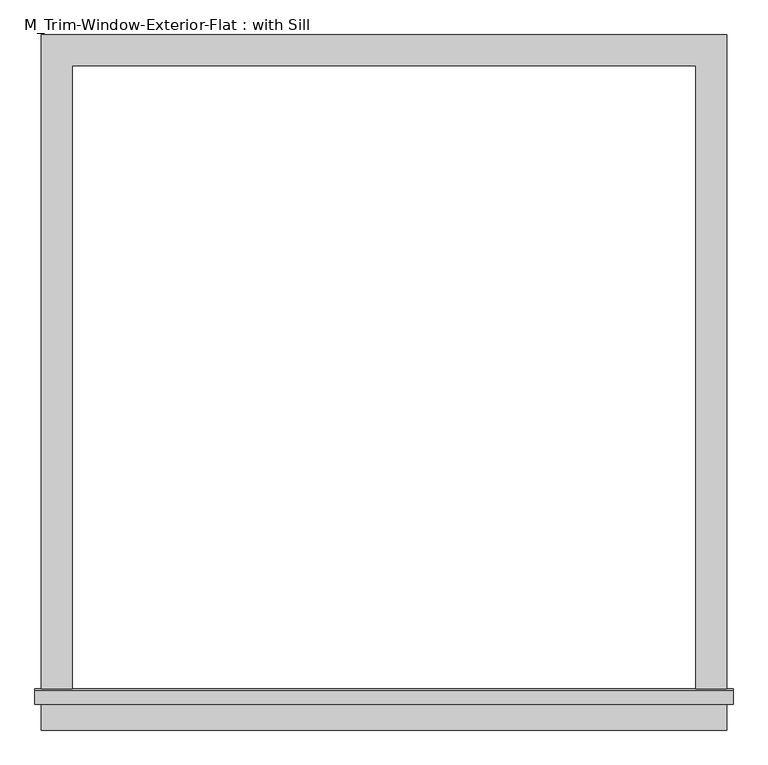
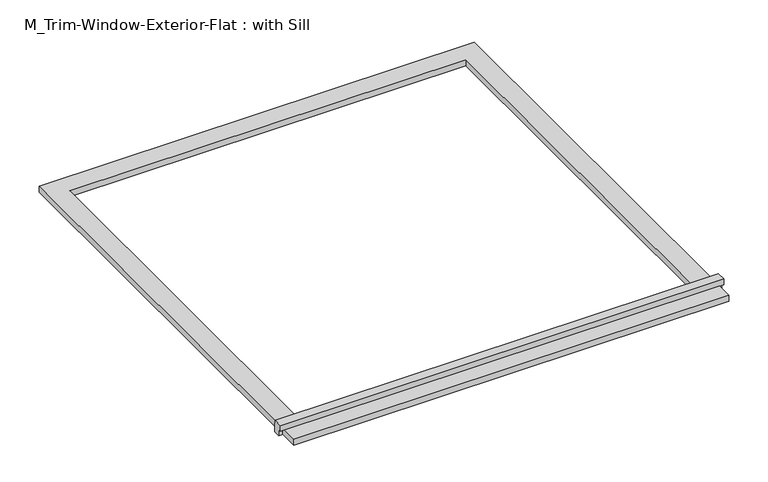
"""IFC4 building model written with IfcOpenShell, lengths in millimetres: proxy geometry, M_Trim-Window-Exterior-Flat : with Sill."""

import ifcopenshell
import ifcopenshell.guid

model = None  # the IFC model being written
_history = None  # IfcOwnerHistory: only IFC2X3 demands one
_inside = {}  # id of a spatial element -> (the spatial element, [elements in it])
_under = {}  # id of a project, library or spatial element -> (it, [spatial elements below it])
_declared = {}  # id of a project -> (the project, [libraries it declares])
_typed = {}  # id of a type object -> (the type object, [elements of that type])
_made_of = {}  # id of a material, layer set ... -> (it, [elements and type objects made of it])


def new_model(schema):
    """Start an empty IFC model of exactly this schema.

    Asked for "IFC4X3", IfcOpenShell would pick the latest addendum, in which some entities
    have other attributes; the version numbers below select the first issue.
    IFC2X3 requires an IfcOwnerHistory on every rooted entity: one is made here for all.
    """
    global model, _history
    if schema == "IFC4X3":
        model = ifcopenshell.file(schema_version=(4, 3, 0, 0))
    else:
        model = ifcopenshell.file(schema=schema)
    _inside.clear()
    _under.clear()
    _declared.clear()
    _typed.clear()
    _made_of.clear()
    _history = None
    if model.schema == "IFC2X3":
        org = make("IfcOrganization", Name="unknown")
        user = make(
            "IfcPersonAndOrganization",
            ThePerson=make("IfcPerson", FamilyName="unknown"),
            TheOrganization=org,
        )
        app = make(
            "IfcApplication",
            ApplicationDeveloper=org,
            Version="unknown",
            ApplicationFullName="unknown",
            ApplicationIdentifier="unknown",
        )
        _history = make(
            "IfcOwnerHistory",
            OwningUser=user,
            OwningApplication=app,
            ChangeAction="ADDED",
            CreationDate=0,
        )
    return model


def make(cls, **values):
    """One entity of the class cls with the attributes given. An attribute that is None is left unset."""
    return model.create_entity(
        cls, **{name: value for name, value in values.items() if value is not None}
    )


def rooted(cls, **values):
    """An entity with a GlobalId (a new one), such as an element, a storey or a relation."""
    return make(cls, GlobalId=ifcopenshell.guid.new(), OwnerHistory=_history, **values)


def si_unit(unit_type, name, prefix=None):
    """IfcSIUnit, for example si_unit("LENGTHUNIT", "METRE", prefix="MILLI")."""
    return make("IfcSIUnit", UnitType=unit_type, Prefix=prefix, Name=name)


def assignment(units):
    """IfcUnitAssignment: the units of a project."""
    return None if units is None else make("IfcUnitAssignment", Units=units)


def point(xyz):
    """IfcCartesianPoint."""
    return None if xyz is None else make("IfcCartesianPoint", Coordinates=xyz)


def direction(xyz):
    """IfcDirection."""
    return None if xyz is None else make("IfcDirection", DirectionRatios=xyz)


def frame(location, z_axis=None, x_axis=None):
    """IfcAxis2Placement3D, a coordinate frame: its origin and axes. An axis left out is left unset."""
    return make(
        "IfcAxis2Placement3D",
        Location=point(location),
        Axis=direction(z_axis),
        RefDirection=direction(x_axis),
    )


def origin():
    """The frame at (0, 0, 0) with its axes left unset."""
    return frame((0.0, 0.0, 0.0))


def origin_with_axes():
    """The frame at (0, 0, 0) with the z axis (0, 0, 1) and the x axis (1, 0, 0) written out."""
    return frame((0.0, 0.0, 0.0), z_axis=(0.0, 0.0, 1.0), x_axis=(1.0, 0.0, 0.0))


def place(relative_to, where):
    """IfcLocalPlacement: puts the frame where relative to a parent placement (None: the world)."""
    return make(
        "IfcLocalPlacement", PlacementRelTo=relative_to, RelativePlacement=where
    )


def context(
    kind, dimensions, precision=None, world=None, true_north=None, identifier=None
):
    """IfcGeometricRepresentationContext, for example the 3D "Model" context."""
    return make(
        "IfcGeometricRepresentationContext",
        ContextIdentifier=identifier,
        ContextType=kind,
        CoordinateSpaceDimension=dimensions,
        Precision=precision,
        WorldCoordinateSystem=world,
        TrueNorth=true_north,
    )


def project(units=None, contexts=None):
    """IfcProject with its units and contexts."""
    return rooted(
        "IfcProject",
        Name="project",
        RepresentationContexts=contexts,
        UnitsInContext=assignment(units),
    )


def spatial(cls, under=None, at=None, **own):
    """A site, building, storey or space (cls), placed at a placement, below another one or the project."""
    s = rooted(cls, ObjectPlacement=at, **own)
    if under is not None:
        _under.setdefault(under.id(), (under, []))[1].append(s)
    return s


def polyline(points):
    """IfcPolyline through the points."""
    return make("IfcPolyline", Points=[point(p) for p in points])


def outline(outer, holes=None, kind="AREA"):
    """IfcArbitraryClosedProfileDef: a profile drawn as a closed curve; with holes, ...WithVoids."""
    if holes is None:
        return make("IfcArbitraryClosedProfileDef", ProfileType=kind, OuterCurve=outer)
    return make(
        "IfcArbitraryProfileDefWithVoids",
        ProfileType=kind,
        OuterCurve=outer,
        InnerCurves=holes,
    )


def extrude(swept, where, along, depth):
    """IfcExtrudedAreaSolid: the profile swept, set in the frame where, extruded along a direction by depth."""
    return make(
        "IfcExtrudedAreaSolid",
        SweptArea=swept,
        Position=where,
        ExtrudedDirection=direction(along),
        Depth=depth,
    )


def shape(context_of_items, identifier, shape_type, items):
    """IfcShapeRepresentation: the items that make up one representation, for example the "Body"."""
    return make(
        "IfcShapeRepresentation",
        ContextOfItems=context_of_items,
        RepresentationIdentifier=identifier,
        RepresentationType=shape_type,
        Items=items,
    )


def source(mapping_origin, context_of_items, identifier, shape_type, items):
    """IfcRepresentationMap: a shape defined once, which mapped items show again and again."""
    return make(
        "IfcRepresentationMap",
        MappingOrigin=mapping_origin,
        MappedRepresentation=shape(context_of_items, identifier, shape_type, items),
    )


def transform(
    local_origin,
    x_axis=None,
    y_axis=None,
    z_axis=None,
    scale=None,
    scale2=None,
    scale3=None,
    uniform=True,
):
    """IfcCartesianTransformationOperator3D, or its non-uniform kind. x_axis, y_axis, z_axis: its Axis1, 2, 3."""
    if uniform:
        return make(
            "IfcCartesianTransformationOperator3D",
            Axis1=direction(x_axis),
            Axis2=direction(y_axis),
            LocalOrigin=point(local_origin),
            Scale=scale,
            Axis3=direction(z_axis),
        )
    return make(
        "IfcCartesianTransformationOperator3DnonUniform",
        Axis1=direction(x_axis),
        Axis2=direction(y_axis),
        LocalOrigin=point(local_origin),
        Scale=scale,
        Axis3=direction(z_axis),
        Scale2=scale2,
        Scale3=scale3,
    )


def mapped(mapping_source, mapping_target):
    """IfcMappedItem: shows the shape of a source again, moved by a transform."""
    return make(
        "IfcMappedItem", MappingSource=mapping_source, MappingTarget=mapping_target
    )


def made_of(thing, what):
    """Note that an element or type object is made of a material, layer set ...; save() writes the relation."""
    if what is not None:
        _made_of.setdefault(what.id(), (what, []))[1].append(thing)
    return thing


def element(
    cls,
    number,
    at=None,
    inside=None,
    cuts=None,
    type_object=None,
    material=None,
    context=None,
    identifier="Body",
    shape_type=None,
    held_by="IfcProductDefinitionShape",
    body=None,
    shapes=None,
    **own,
):
    """One element of the class cls, such as IfcWall. Its Tag is "e" and its number.

    at: its placement. inside: the storey or other place that contains it. cuts: it is an
    opening in that element (IfcRelVoidsElement). A single representation is given by context,
    identifier, shape_type and body (its items); several are given by shapes. held_by: the class
    of the entity that holds the representations. save() writes the other relations.
    """
    e = rooted(cls, Tag="e%d" % number, ObjectPlacement=at, **own)
    if body is not None:
        shapes = [shape(context, identifier, shape_type, body)]
    if shapes is not None:
        e.Representation = make(held_by, Representations=shapes)
    if inside is not None:
        _inside.setdefault(inside.id(), (inside, []))[1].append(e)
    if cuts is not None:
        rooted(
            "IfcRelVoidsElement", RelatingBuildingElement=cuts, RelatedOpeningElement=e
        )
    if type_object is not None:
        _typed.setdefault(type_object.id(), (type_object, []))[1].append(e)
    return made_of(e, material)


def aggregate(whole, parts):
    """IfcRelAggregates: a whole, such as a stair, and the parts it consists of."""
    return rooted("IfcRelAggregates", RelatingObject=whole, RelatedObjects=parts)


def save(model, path):
    """Write the relations noted so far, then the file.

    IfcRelAggregates (storeys below a building ...), IfcRelContainedInSpatialStructure (elements
    in a storey), IfcRelDefinesByType, IfcRelAssociatesMaterial and IfcRelDeclares: one each for
    every whole, place, type object, material and project.
    """
    for whole, parts in _under.values():
        aggregate(whole, parts)
    for where, things in _inside.values():
        rooted(
            "IfcRelContainedInSpatialStructure",
            RelatedElements=things,
            RelatingStructure=where,
        )
    for kind, things in _typed.values():
        rooted("IfcRelDefinesByType", RelatedObjects=things, RelatingType=kind)
    for what, things in _made_of.values():
        rooted("IfcRelAssociatesMaterial", RelatedObjects=things, RelatingMaterial=what)
    for by, libraries in _declared.values():
        rooted("IfcRelDeclares", RelatingContext=by, RelatedDefinitions=libraries)
    model.write(path)


def m_trim_window_exterior_flat_with_sill_9a9e3a74(model_context):
    return source(origin(), model_context, "Body", "SweptSolid", [
        extrude(outline(polyline([(669.6, -1239.6323709), (669.6, -1299.6323709), (-669.6, -1299.6323709), (-669.6, -1239.6323709), (669.6, -1239.6323709)])), origin_with_axes(), (0.0, 0.0, 1.0), 19.05),
        extrude(outline(polyline([(-1249.2, 38.1), (-1221.6580645, 38.1), (-1219.2, 19.05), (-1219.2, 0.0), (-1239.6323709, 0.0), (-1239.6323709, 19.05), (-1249.2, 19.05), (-1249.2, 38.1)])), frame((-682.3, 0.0, 0.0), z_axis=(1.0, 0.0, 0.0), x_axis=(0.0, 1.0, 0.0)), (0.0, 0.0, 1.0), 1364.6),
        extrude(outline(polyline([(-669.6, 60.0), (669.6, 60.0), (669.6, -1219.2), (609.6, -1219.2), (609.6, 0.0), (-609.6, 0.0), (-609.6, -1219.2), (-669.6, -1219.2), (-669.6, 60.0)])), origin_with_axes(), (0.0, 0.0, 1.0), 19.05),
    ])


if __name__ == "__main__":
    model = new_model("IFC4")
    model_context = context("Model", 3, world=origin())
    ifc_project = project(units=[si_unit("LENGTHUNIT", "METRE", prefix="MILLI")], contexts=[model_context])
    site = spatial("IfcSite", under=ifc_project)
    building = spatial("IfcBuilding", under=site)
    placement = place(None, origin())
    m_trim_window_exterior_flat_with_sill_shape = m_trim_window_exterior_flat_with_sill_9a9e3a74(model_context)
    element("IfcBuildingElementProxy", 1, Name="M_Trim-Window-Exterior-Flat : with Sill", ObjectType="M_Trim-Window-Exterior-Flat : with Sill", at=placement, inside=building, context=model_context, shape_type="MappedRepresentation", body=[
        mapped(m_trim_window_exterior_flat_with_sill_shape, transform((0.0, 0.0, 0.0), x_axis=(1.0, 0.0, 0.0), y_axis=(0.0, 1.0, 0.0), z_axis=(0.0, 0.0, 1.0))),
    ])
    save(model, "model.ifc")

# Revit data of these elements
# Type "M_Trim-Window-Exterior-Flat : with Sill"
#   Trim Width = 0' - 2.3622"
#   Trim Thickness_Picture Frame = 0' - 1.1811"
#   Trim Thickness_with Sill = 0' - 0 3/4"
#   Sill Thickness = 0' - 1.1811"
#   Opening Width [instance default] = 1' - 11.62205"
#   Opening Height [instance default] = 2' - 11.43307"
#   Default Elevation = 3' - 11.24409"
#   Sill = yes
#   Picture Frame = no
#   Trim Material [instance default] = none
# Element 1 (IfcBuildingElementProxy, "M_Trim-Window-Exterior-Flat : with Sill")
#   Opening Width = 4' - 0"
#   Opening Height = 4' - 0"
#   Trim Material = Clad - White
#   Materials on its faces: "Clad - White"
# Materials
#   "Clad - White": class "Wood", colour RGB 242 242 238, transparency 0, Cost = 0
